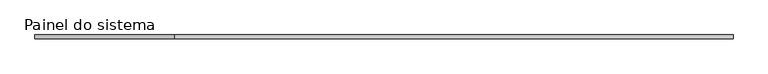
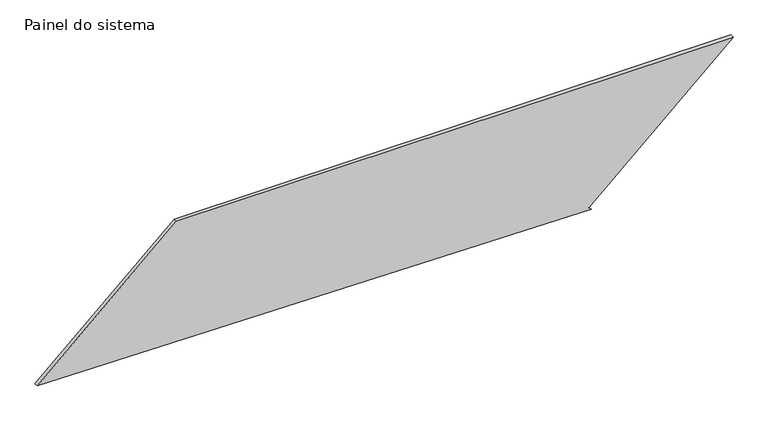
"""IFC4 building model written with IfcOpenShell, lengths in millimetres: plate geometry, Painel do sistema : Envidraçado."""

import ifcopenshell
import ifcopenshell.guid

model = None  # the IFC model being written
_history = None  # IfcOwnerHistory: only IFC2X3 demands one
_inside = {}  # id of a spatial element -> (the spatial element, [elements in it])
_under = {}  # id of a project, library or spatial element -> (it, [spatial elements below it])
_declared = {}  # id of a project -> (the project, [libraries it declares])
_typed = {}  # id of a type object -> (the type object, [elements of that type])
_made_of = {}  # id of a material, layer set ... -> (it, [elements and type objects made of it])


def new_model(schema):
    """Start an empty IFC model of exactly this schema.

    Asked for "IFC4X3", IfcOpenShell would pick the latest addendum, in which some entities
    have other attributes; the version numbers below select the first issue.
    IFC2X3 requires an IfcOwnerHistory on every rooted entity: one is made here for all.
    """
    global model, _history
    if schema == "IFC4X3":
        model = ifcopenshell.file(schema_version=(4, 3, 0, 0))
    else:
        model = ifcopenshell.file(schema=schema)
    _inside.clear()
    _under.clear()
    _declared.clear()
    _typed.clear()
    _made_of.clear()
    _history = None
    if model.schema == "IFC2X3":
        org = make("IfcOrganization", Name="unknown")
        user = make(
            "IfcPersonAndOrganization",
            ThePerson=make("IfcPerson", FamilyName="unknown"),
            TheOrganization=org,
        )
        app = make(
            "IfcApplication",
            ApplicationDeveloper=org,
            Version="unknown",
            ApplicationFullName="unknown",
            ApplicationIdentifier="unknown",
        )
        _history = make(
            "IfcOwnerHistory",
            OwningUser=user,
            OwningApplication=app,
            ChangeAction="ADDED",
            CreationDate=0,
        )
    return model


def make(cls, **values):
    """One entity of the class cls with the attributes given. An attribute that is None is left unset."""
    return model.create_entity(
        cls, **{name: value for name, value in values.items() if value is not None}
    )


def rooted(cls, **values):
    """An entity with a GlobalId (a new one), such as an element, a storey or a relation."""
    return make(cls, GlobalId=ifcopenshell.guid.new(), OwnerHistory=_history, **values)


def si_unit(unit_type, name, prefix=None):
    """IfcSIUnit, for example si_unit("LENGTHUNIT", "METRE", prefix="MILLI")."""
    return make("IfcSIUnit", UnitType=unit_type, Prefix=prefix, Name=name)


def assignment(units):
    """IfcUnitAssignment: the units of a project."""
    return None if units is None else make("IfcUnitAssignment", Units=units)


def point(xyz):
    """IfcCartesianPoint."""
    return None if xyz is None else make("IfcCartesianPoint", Coordinates=xyz)


def direction(xyz):
    """IfcDirection."""
    return None if xyz is None else make("IfcDirection", DirectionRatios=xyz)


def frame(location, z_axis=None, x_axis=None):
    """IfcAxis2Placement3D, a coordinate frame: its origin and axes. An axis left out is left unset."""
    return make(
        "IfcAxis2Placement3D",
        Location=point(location),
        Axis=direction(z_axis),
        RefDirection=direction(x_axis),
    )


def origin():
    """The frame at (0, 0, 0) with its axes left unset."""
    return frame((0.0, 0.0, 0.0))


def place(relative_to, where):
    """IfcLocalPlacement: puts the frame where relative to a parent placement (None: the world)."""
    return make(
        "IfcLocalPlacement", PlacementRelTo=relative_to, RelativePlacement=where
    )


def context(
    kind, dimensions, precision=None, world=None, true_north=None, identifier=None
):
    """IfcGeometricRepresentationContext, for example the 3D "Model" context."""
    return make(
        "IfcGeometricRepresentationContext",
        ContextIdentifier=identifier,
        ContextType=kind,
        CoordinateSpaceDimension=dimensions,
        Precision=precision,
        WorldCoordinateSystem=world,
        TrueNorth=true_north,
    )


def project(units=None, contexts=None):
    """IfcProject with its units and contexts."""
    return rooted(
        "IfcProject",
        Name="project",
        RepresentationContexts=contexts,
        UnitsInContext=assignment(units),
    )


def spatial(cls, under=None, at=None, **own):
    """A site, building, storey or space (cls), placed at a placement, below another one or the project."""
    s = rooted(cls, ObjectPlacement=at, **own)
    if under is not None:
        _under.setdefault(under.id(), (under, []))[1].append(s)
    return s


def polyline(points):
    """IfcPolyline through the points."""
    return make("IfcPolyline", Points=[point(p) for p in points])


def outline(outer, holes=None, kind="AREA"):
    """IfcArbitraryClosedProfileDef: a profile drawn as a closed curve; with holes, ...WithVoids."""
    if holes is None:
        return make("IfcArbitraryClosedProfileDef", ProfileType=kind, OuterCurve=outer)
    return make(
        "IfcArbitraryProfileDefWithVoids",
        ProfileType=kind,
        OuterCurve=outer,
        InnerCurves=holes,
    )


def extrude(swept, where, along, depth):
    """IfcExtrudedAreaSolid: the profile swept, set in the frame where, extruded along a direction by depth."""
    return make(
        "IfcExtrudedAreaSolid",
        SweptArea=swept,
        Position=where,
        ExtrudedDirection=direction(along),
        Depth=depth,
    )


def shape(context_of_items, identifier, shape_type, items):
    """IfcShapeRepresentation: the items that make up one representation, for example the "Body"."""
    return make(
        "IfcShapeRepresentation",
        ContextOfItems=context_of_items,
        RepresentationIdentifier=identifier,
        RepresentationType=shape_type,
        Items=items,
    )


def source(mapping_origin, context_of_items, identifier, shape_type, items):
    """IfcRepresentationMap: a shape defined once, which mapped items show again and again."""
    return make(
        "IfcRepresentationMap",
        MappingOrigin=mapping_origin,
        MappedRepresentation=shape(context_of_items, identifier, shape_type, items),
    )


def transform(
    local_origin,
    x_axis=None,
    y_axis=None,
    z_axis=None,
    scale=None,
    scale2=None,
    scale3=None,
    uniform=True,
):
    """IfcCartesianTransformationOperator3D, or its non-uniform kind. x_axis, y_axis, z_axis: its Axis1, 2, 3."""
    if uniform:
        return make(
            "IfcCartesianTransformationOperator3D",
            Axis1=direction(x_axis),
            Axis2=direction(y_axis),
            LocalOrigin=point(local_origin),
            Scale=scale,
            Axis3=direction(z_axis),
        )
    return make(
        "IfcCartesianTransformationOperator3DnonUniform",
        Axis1=direction(x_axis),
        Axis2=direction(y_axis),
        LocalOrigin=point(local_origin),
        Scale=scale,
        Axis3=direction(z_axis),
        Scale2=scale2,
        Scale3=scale3,
    )


def mapped(mapping_source, mapping_target):
    """IfcMappedItem: shows the shape of a source again, moved by a transform."""
    return make(
        "IfcMappedItem", MappingSource=mapping_source, MappingTarget=mapping_target
    )


def made_of(thing, what):
    """Note that an element or type object is made of a material, layer set ...; save() writes the relation."""
    if what is not None:
        _made_of.setdefault(what.id(), (what, []))[1].append(thing)
    return thing


def element(
    cls,
    number,
    at=None,
    inside=None,
    cuts=None,
    type_object=None,
    material=None,
    context=None,
    identifier="Body",
    shape_type=None,
    held_by="IfcProductDefinitionShape",
    body=None,
    shapes=None,
    **own,
):
    """One element of the class cls, such as IfcWall. Its Tag is "e" and its number.

    at: its placement. inside: the storey or other place that contains it. cuts: it is an
    opening in that element (IfcRelVoidsElement). A single representation is given by context,
    identifier, shape_type and body (its items); several are given by shapes. held_by: the class
    of the entity that holds the representations. save() writes the other relations.
    """
    e = rooted(cls, Tag="e%d" % number, ObjectPlacement=at, **own)
    if body is not None:
        shapes = [shape(context, identifier, shape_type, body)]
    if shapes is not None:
        e.Representation = make(held_by, Representations=shapes)
    if inside is not None:
        _inside.setdefault(inside.id(), (inside, []))[1].append(e)
    if cuts is not None:
        rooted(
            "IfcRelVoidsElement", RelatingBuildingElement=cuts, RelatedOpeningElement=e
        )
    if type_object is not None:
        _typed.setdefault(type_object.id(), (type_object, []))[1].append(e)
    return made_of(e, material)


def aggregate(whole, parts):
    """IfcRelAggregates: a whole, such as a stair, and the parts it consists of."""
    return rooted("IfcRelAggregates", RelatingObject=whole, RelatedObjects=parts)


def save(model, path):
    """Write the relations noted so far, then the file.

    IfcRelAggregates (storeys below a building ...), IfcRelContainedInSpatialStructure (elements
    in a storey), IfcRelDefinesByType, IfcRelAssociatesMaterial and IfcRelDeclares: one each for
    every whole, place, type object, material and project.
    """
    for whole, parts in _under.values():
        aggregate(whole, parts)
    for where, things in _inside.values():
        rooted(
            "IfcRelContainedInSpatialStructure",
            RelatedElements=things,
            RelatingStructure=where,
        )
    for kind, things in _typed.values():
        rooted("IfcRelDefinesByType", RelatedObjects=things, RelatingType=kind)
    for what, things in _made_of.values():
        rooted("IfcRelAssociatesMaterial", RelatedObjects=things, RelatingMaterial=what)
    for by, libraries in _declared.values():
        rooted("IfcRelDeclares", RelatingContext=by, RelatedDefinitions=libraries)
    model.write(path)


def painel_do_sistema_6486837b(model_context):
    return source(origin(), model_context, "Body", "SweptSolid", [
        extrude(outline(polyline([(0.0, 1410.803261), (18.5968466, 1394.0952601), (907.3270606, 2383.296754), (907.3270606, -1428.6927274), (49.6803162, -2383.296754), (0.0, 1410.803261)])), frame((0.0, 24.5, 0.0), z_axis=(0.0, 1.0, 0.0), x_axis=(0.0, 0.0, 1.0)), (0.0, 0.0, 1.0), 25.0),
    ])


if __name__ == "__main__":
    model = new_model("IFC4")
    model_context = context("Model", 3, world=origin())
    ifc_project = project(units=[si_unit("LENGTHUNIT", "METRE", prefix="MILLI")], contexts=[model_context])
    site = spatial("IfcSite", under=ifc_project)
    building = spatial("IfcBuilding", under=site)
    placement = place(None, origin())
    painel_do_sistema_shape = painel_do_sistema_6486837b(model_context)
    element("IfcPlate", 1, ObjectType="Painel do sistema : Envidraçado", at=placement, inside=building, context=model_context, shape_type="MappedRepresentation", body=[
        mapped(painel_do_sistema_shape, transform((0.0, 0.0, 0.0), x_axis=(1.0, 0.0, 0.0), y_axis=(0.0, 1.0, 0.0), z_axis=(0.0, 0.0, 1.0))),
    ])
    save(model, "model.ifc")

# Revit data of these elements
# Type "Painel do sistema : Envidraçado"
#   Construction Type Id = "GSP4R"
#   Analytic Construction = "Vidraça única Pilkington 1/8 pol"
#   Visual Light Transmittance = 0.9
#   Solar Heat Gain Coefficient = 0.86
#   Heat Transfer Coefficient (U) = 6.7069 W/(m²·K)
# Element 1 (IfcPlate, "Painel do sistema : Envidraçado")
#   Materials on its faces: "Vidro"
# Materials
#   "Vidro": class "Vidro", colour RGB 0 128 192, transparency 0.9, Description = "Vidro de sílica", Cost = 0
